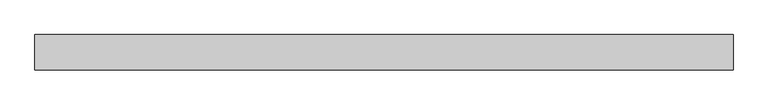
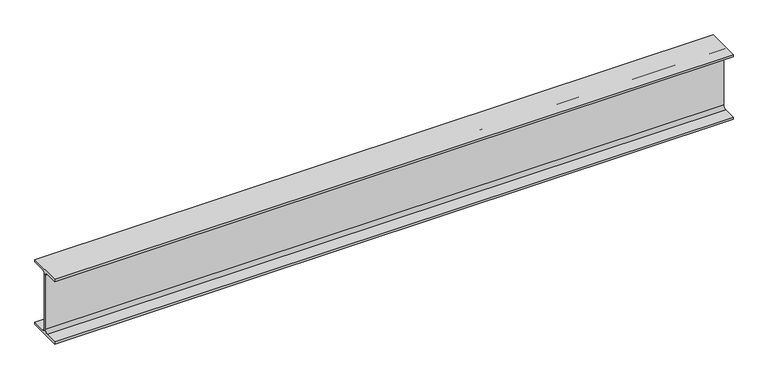
"""IFC4 building model written with IfcOpenShell, lengths in millimetres: beam geometry, 0912_Steel Framing_H-KSD3502 : H_SB_ASB_H-250x125x6x9."""

from ifc_helpers import new_model, si_unit, point, frame, frame_2d, origin, place, context, project, spatial, polyline, circle_curve, trimmed, segment, composite_curve, outline, extrude, source, transform, mapped, element, save


def beam_e193e52b(model_context):
    return source(origin(), model_context, "Body", "SweptSolid", [
        extrude(outline(composite_curve([segment(polyline([(62.5, -116.0), (62.5, -125.0), (-62.5, -125.0), (-62.5, -116.0), (-15.0, -116.0)]), True, "CONTINUOUS"), segment(trimmed(circle_curve(frame_2d((-15.0, -104.0)), 12.0), [point((-15.0, -116.0))], [point((-3.0, -104.0))], True, "CARTESIAN"), True, "CONTINUOUS"), segment(polyline([(-3.0, -104.0), (-3.0, 104.0)]), True, "CONTINUOUS"), segment(trimmed(circle_curve(frame_2d((-15.0, 104.0)), 12.0), [point((-3.0, 104.0))], [point((-15.0, 116.0))], True, "CARTESIAN"), True, "CONTINUOUS"), segment(polyline([(-15.0, 116.0), (-62.5, 116.0), (-62.5, 125.0), (62.5, 125.0), (62.5, 116.0), (15.0, 116.0)]), True, "CONTINUOUS"), segment(trimmed(circle_curve(frame_2d((15.0, 104.0)), 12.0), [point((15.0, 116.0))], [point((3.0, 104.0))], True, "CARTESIAN"), True, "CONTINUOUS"), segment(polyline([(3.0, 104.0), (3.0, -104.0)]), True, "CONTINUOUS"), segment(trimmed(circle_curve(frame_2d((15.0, -104.0)), 12.0), [point((3.0, -104.0))], [point((15.0, -116.0))], True, "CARTESIAN"), True, "CONTINUOUS"), segment(polyline([(15.0, -116.0), (62.5, -116.0)]), True, "CONTINUOUS")], self_intersect=False)), frame((-1137.3, 0.0, 0.0), z_axis=(1.0, 0.0, 0.0), x_axis=(0.0, 1.0, 0.0)), (0.0, 0.0, 1.0), 2474.6),
    ])


if __name__ == "__main__":
    model = new_model("IFC4")
    model_context = context("Model", 3, world=origin())
    ifc_project = project(units=[si_unit("LENGTHUNIT", "METRE", prefix="MILLI")], contexts=[model_context])
    site = spatial("IfcSite", under=ifc_project)
    building = spatial("IfcBuilding", under=site)
    placement = place(None, origin())
    beam_shape = beam_e193e52b(model_context)
    element("IfcBeam", 1, ObjectType="0912_Steel Framing_H-KSD3502 : H_SB_ASB_H-250x125x6x9", at=placement, inside=building, context=model_context, shape_type="MappedRepresentation", body=[
        mapped(beam_shape, transform((0.0, 0.0, 0.0), x_axis=(1.0, 0.0, 0.0), y_axis=(0.0, 1.0, 0.0), z_axis=(0.0, 0.0, 1.0))),
    ])
    save(model, "model.ifc")

# Revit data of these elements
# Type "0912_Steel Framing_H-KSD3502 : H_SB_ASB_H-250x125x6x9"
#   H_WM Code_1 = "S01AA003-00001 | Main Steel Structure Fabrication Work | Shelter/Building | Light Steel - Standard (30KG/M>Weight) | Material: (   )"
#   H_WM Code_2 = "S03AA029-00001 | Main Steel Structure Erection Work | Shelter/Building | Light Steel (30KG/M>Weight) | Material: (   )"
#   H_WM Code_3 = "S01AA010-00001 | Main Steel Structure Fabrication Work | Shelter/Building | Steel Painting/Coating | for Non-Fireproofed Steel Surface, Surface Preparation, Primer, Second & Final Coat | Material: (   )"
#   H_Q'ty Cal Type Tag = "SB-Q2"
#   Width = 12.5 cm
#   Web Thickness = 0.6 cm
#   Web Fillet = 1.2 cm
#   Warping Constant = 42539.8 cm⁶
#   W = 0
#   Torsional Moment of Inertia = 7.8102 cm⁴
#   Section Area = 37.66 cm²
#   Plastic Modulus weak axis = 73.1 cm³
#   Plastic Modulus strong axis = 366.0 cm³
#   Perimeter = 0.97 m²/m
#   Nominal Weight = 29.60 kgf/m
#   Moment of Inertia weak axis = 294.00 cm⁴
#   Moment of Inertia strong axis = 4050.00 cm⁴
#   Height = 25.0 cm
#   Flange Thickness = 0.9 cm
#   Elastic Modulus weak axis = 47.0 cm³
#   Elastic Modulus strong axis = 324.0 cm³
#   Centroid Vertical = 12.5 cm
#   Centroid Horizontal = 6.25 cm
#   Ix = 40500000
#   Length [instance default] = 1.5240 m
#   Zx = 366000
#   b = 0.1250 m
#   h = 0.2500 m
#   r = 0.0120 m
#   s = 0.0060 m
#   t = 0.0090 m
#   A = 0.003766 m²
#   Structural Material [instance default] = Steel, 45-345
#   Assembly Code = ""
# Element 1 (IfcBeam, "0912_Steel Framing_H-KSD3502 : H_SB_ASB_H-250x125x6x9")
#   Structural Material = none
# Materials
#   "Steel, 45-345": class "Metal", colour RGB 189 187 185, transparency 0, Description = "Steel 345 MPa", Cost = 0
